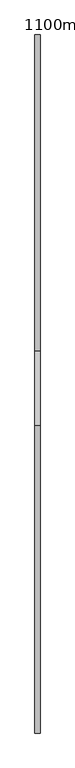
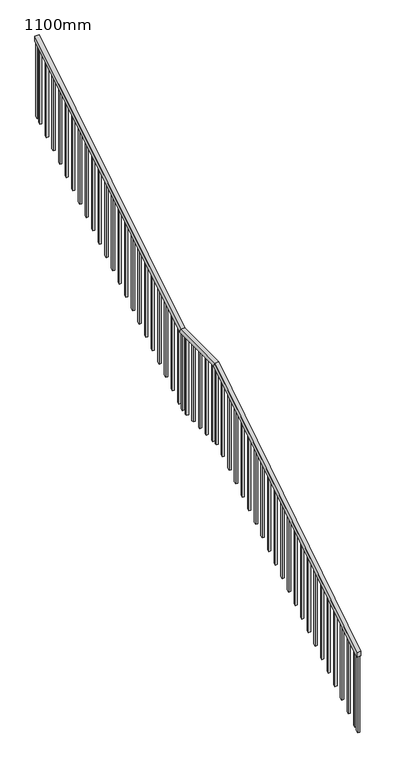
"""IFC4 building model written with IfcOpenShell, lengths in millimetres: railing geometry, 1100mm."""

import ifcopenshell
import ifcopenshell.guid

model = None  # the IFC model being written
_history = None  # IfcOwnerHistory: only IFC2X3 demands one
_inside = {}  # id of a spatial element -> (the spatial element, [elements in it])
_under = {}  # id of a project, library or spatial element -> (it, [spatial elements below it])
_declared = {}  # id of a project -> (the project, [libraries it declares])
_typed = {}  # id of a type object -> (the type object, [elements of that type])
_made_of = {}  # id of a material, layer set ... -> (it, [elements and type objects made of it])


def new_model(schema):
    """Start an empty IFC model of exactly this schema.

    Asked for "IFC4X3", IfcOpenShell would pick the latest addendum, in which some entities
    have other attributes; the version numbers below select the first issue.
    IFC2X3 requires an IfcOwnerHistory on every rooted entity: one is made here for all.
    """
    global model, _history
    if schema == "IFC4X3":
        model = ifcopenshell.file(schema_version=(4, 3, 0, 0))
    else:
        model = ifcopenshell.file(schema=schema)
    _inside.clear()
    _under.clear()
    _declared.clear()
    _typed.clear()
    _made_of.clear()
    _history = None
    if model.schema == "IFC2X3":
        org = make("IfcOrganization", Name="unknown")
        user = make(
            "IfcPersonAndOrganization",
            ThePerson=make("IfcPerson", FamilyName="unknown"),
            TheOrganization=org,
        )
        app = make(
            "IfcApplication",
            ApplicationDeveloper=org,
            Version="unknown",
            ApplicationFullName="unknown",
            ApplicationIdentifier="unknown",
        )
        _history = make(
            "IfcOwnerHistory",
            OwningUser=user,
            OwningApplication=app,
            ChangeAction="ADDED",
            CreationDate=0,
        )
    return model


def make(cls, **values):
    """One entity of the class cls with the attributes given. An attribute that is None is left unset."""
    return model.create_entity(
        cls, **{name: value for name, value in values.items() if value is not None}
    )


def rooted(cls, **values):
    """An entity with a GlobalId (a new one), such as an element, a storey or a relation."""
    return make(cls, GlobalId=ifcopenshell.guid.new(), OwnerHistory=_history, **values)


def si_unit(unit_type, name, prefix=None):
    """IfcSIUnit, for example si_unit("LENGTHUNIT", "METRE", prefix="MILLI")."""
    return make("IfcSIUnit", UnitType=unit_type, Prefix=prefix, Name=name)


def assignment(units):
    """IfcUnitAssignment: the units of a project."""
    return None if units is None else make("IfcUnitAssignment", Units=units)


def point(xyz):
    """IfcCartesianPoint."""
    return None if xyz is None else make("IfcCartesianPoint", Coordinates=xyz)


def direction(xyz):
    """IfcDirection."""
    return None if xyz is None else make("IfcDirection", DirectionRatios=xyz)


def frame(location, z_axis=None, x_axis=None):
    """IfcAxis2Placement3D, a coordinate frame: its origin and axes. An axis left out is left unset."""
    return make(
        "IfcAxis2Placement3D",
        Location=point(location),
        Axis=direction(z_axis),
        RefDirection=direction(x_axis),
    )


def origin():
    """The frame at (0, 0, 0) with its axes left unset."""
    return frame((0.0, 0.0, 0.0))


def place(relative_to, where):
    """IfcLocalPlacement: puts the frame where relative to a parent placement (None: the world)."""
    return make(
        "IfcLocalPlacement", PlacementRelTo=relative_to, RelativePlacement=where
    )


def context(
    kind, dimensions, precision=None, world=None, true_north=None, identifier=None
):
    """IfcGeometricRepresentationContext, for example the 3D "Model" context."""
    return make(
        "IfcGeometricRepresentationContext",
        ContextIdentifier=identifier,
        ContextType=kind,
        CoordinateSpaceDimension=dimensions,
        Precision=precision,
        WorldCoordinateSystem=world,
        TrueNorth=true_north,
    )


def project(units=None, contexts=None):
    """IfcProject with its units and contexts."""
    return rooted(
        "IfcProject",
        Name="project",
        RepresentationContexts=contexts,
        UnitsInContext=assignment(units),
    )


def spatial(cls, under=None, at=None, **own):
    """A site, building, storey or space (cls), placed at a placement, below another one or the project."""
    s = rooted(cls, ObjectPlacement=at, **own)
    if under is not None:
        _under.setdefault(under.id(), (under, []))[1].append(s)
    return s


def polyline(points):
    """IfcPolyline through the points."""
    return make("IfcPolyline", Points=[point(p) for p in points])


def outline(outer, holes=None, kind="AREA"):
    """IfcArbitraryClosedProfileDef: a profile drawn as a closed curve; with holes, ...WithVoids."""
    if holes is None:
        return make("IfcArbitraryClosedProfileDef", ProfileType=kind, OuterCurve=outer)
    return make(
        "IfcArbitraryProfileDefWithVoids",
        ProfileType=kind,
        OuterCurve=outer,
        InnerCurves=holes,
    )


def extrude(swept, where, along, depth):
    """IfcExtrudedAreaSolid: the profile swept, set in the frame where, extruded along a direction by depth."""
    return make(
        "IfcExtrudedAreaSolid",
        SweptArea=swept,
        Position=where,
        ExtrudedDirection=direction(along),
        Depth=depth,
    )


def faces_of(points, faces, orient=None, outer=None):
    """IfcFace entities. A face is a list of loops; a loop is a list of indices into points, from 0.

    orient and outer hold one flag for each loop. By default every Orientation is true, the
    first loop of a face is its IfcFaceOuterBound and the others are IfcFaceBound.
    """
    made = []
    for i, loops in enumerate(faces):
        bounds = []
        for j, loop in enumerate(loops):
            is_outer = j == 0 if outer is None else outer[i][j]
            bounds.append(
                make(
                    "IfcFaceOuterBound" if is_outer else "IfcFaceBound",
                    Bound=make("IfcPolyLoop", Polygon=[points[k] for k in loop]),
                    Orientation=True if orient is None else orient[i][j],
                )
            )
        made.append(make("IfcFace", Bounds=bounds))
    return made


def faceted_brep(points, faces, orient=None, outer=None, voids=None):
    """IfcFacetedBrep: a solid bounded by flat faces; with voids (closed shells), ...WithVoids."""
    shared = [point(p) for p in points]
    hull = make("IfcClosedShell", CfsFaces=faces_of(shared, faces, orient, outer))
    if voids is None:
        return make("IfcFacetedBrep", Outer=hull)
    return make(
        "IfcFacetedBrepWithVoids",
        Outer=hull,
        Voids=[
            make(cls, CfsFaces=faces_of(shared, fs, o, b)) for cls, fs, o, b in voids
        ],
    )


def shape(context_of_items, identifier, shape_type, items):
    """IfcShapeRepresentation: the items that make up one representation, for example the "Body"."""
    return make(
        "IfcShapeRepresentation",
        ContextOfItems=context_of_items,
        RepresentationIdentifier=identifier,
        RepresentationType=shape_type,
        Items=items,
    )


def source(mapping_origin, context_of_items, identifier, shape_type, items):
    """IfcRepresentationMap: a shape defined once, which mapped items show again and again."""
    return make(
        "IfcRepresentationMap",
        MappingOrigin=mapping_origin,
        MappedRepresentation=shape(context_of_items, identifier, shape_type, items),
    )


def transform(
    local_origin,
    x_axis=None,
    y_axis=None,
    z_axis=None,
    scale=None,
    scale2=None,
    scale3=None,
    uniform=True,
):
    """IfcCartesianTransformationOperator3D, or its non-uniform kind. x_axis, y_axis, z_axis: its Axis1, 2, 3."""
    if uniform:
        return make(
            "IfcCartesianTransformationOperator3D",
            Axis1=direction(x_axis),
            Axis2=direction(y_axis),
            LocalOrigin=point(local_origin),
            Scale=scale,
            Axis3=direction(z_axis),
        )
    return make(
        "IfcCartesianTransformationOperator3DnonUniform",
        Axis1=direction(x_axis),
        Axis2=direction(y_axis),
        LocalOrigin=point(local_origin),
        Scale=scale,
        Axis3=direction(z_axis),
        Scale2=scale2,
        Scale3=scale3,
    )


def mapped(mapping_source, mapping_target):
    """IfcMappedItem: shows the shape of a source again, moved by a transform."""
    return make(
        "IfcMappedItem", MappingSource=mapping_source, MappingTarget=mapping_target
    )


def made_of(thing, what):
    """Note that an element or type object is made of a material, layer set ...; save() writes the relation."""
    if what is not None:
        _made_of.setdefault(what.id(), (what, []))[1].append(thing)
    return thing


def element(
    cls,
    number,
    at=None,
    inside=None,
    cuts=None,
    type_object=None,
    material=None,
    context=None,
    identifier="Body",
    shape_type=None,
    held_by="IfcProductDefinitionShape",
    body=None,
    shapes=None,
    **own,
):
    """One element of the class cls, such as IfcWall. Its Tag is "e" and its number.

    at: its placement. inside: the storey or other place that contains it. cuts: it is an
    opening in that element (IfcRelVoidsElement). A single representation is given by context,
    identifier, shape_type and body (its items); several are given by shapes. held_by: the class
    of the entity that holds the representations. save() writes the other relations.
    """
    e = rooted(cls, Tag="e%d" % number, ObjectPlacement=at, **own)
    if body is not None:
        shapes = [shape(context, identifier, shape_type, body)]
    if shapes is not None:
        e.Representation = make(held_by, Representations=shapes)
    if inside is not None:
        _inside.setdefault(inside.id(), (inside, []))[1].append(e)
    if cuts is not None:
        rooted(
            "IfcRelVoidsElement", RelatingBuildingElement=cuts, RelatedOpeningElement=e
        )
    if type_object is not None:
        _typed.setdefault(type_object.id(), (type_object, []))[1].append(e)
    return made_of(e, material)


def aggregate(whole, parts):
    """IfcRelAggregates: a whole, such as a stair, and the parts it consists of."""
    return rooted("IfcRelAggregates", RelatingObject=whole, RelatedObjects=parts)


def save(model, path):
    """Write the relations noted so far, then the file.

    IfcRelAggregates (storeys below a building ...), IfcRelContainedInSpatialStructure (elements
    in a storey), IfcRelDefinesByType, IfcRelAssociatesMaterial and IfcRelDeclares: one each for
    every whole, place, type object, material and project.
    """
    for whole, parts in _under.values():
        aggregate(whole, parts)
    for where, things in _inside.values():
        rooted(
            "IfcRelContainedInSpatialStructure",
            RelatedElements=things,
            RelatingStructure=where,
        )
    for kind, things in _typed.values():
        rooted("IfcRelDefinesByType", RelatedObjects=things, RelatingType=kind)
    for what, things in _made_of.values():
        rooted("IfcRelAssociatesMaterial", RelatedObjects=things, RelatingMaterial=what)
    for by, libraries in _declared.values():
        rooted("IfcRelDeclares", RelatingContext=by, RelatedDefinitions=libraries)
    model.write(path)


def railing_1100mm_2fb11b6b(model_context):
    return source(origin(), model_context, "Body", "SolidModel", [
        faceted_brep([(-22150.0159097, -6684.456375, 1268.797954), (-22150.0159097, -6684.456375, 1209.4512039), (-22100.0159097, -6684.456375, 1209.4512039), (-22100.0159097, -6684.456375, 1268.797954), (-22150.0159097, -3684.456375, 3186.9565217), (-22150.0159097, -3669.8380579, 3136.9565217), (-22100.0159097, -3669.8380579, 3136.9565217), (-22100.0159097, -3684.456375, 3186.9565217), (-22150.0159097, -2964.456375, 3186.9565217), (-22150.0159097, -2950.192194, 3136.9565217), (-22100.0159097, -2950.192194, 3136.9565217), (-22100.0159097, -2964.456375, 3186.9565217), (-22150.0159097, 115.543625, 5100.0), (-22100.0159097, 115.543625, 5100.0), (-22100.0159097, 115.543625, 5041.1402603), (-22150.0159097, 115.543625, 5041.1402603)], [[[0, 1, 2, 3]], [[1, 0, 4, 5]], [[2, 1, 5, 6]], [[3, 2, 6, 7]], [[0, 3, 7, 4]], [[5, 4, 8, 9]], [[6, 5, 9, 10]], [[7, 6, 10, 11]], [[4, 7, 11, 8]], [[12, 13, 14, 15]], [[9, 8, 12, 15]], [[10, 9, 15, 14]], [[11, 10, 14, 13]], [[8, 11, 13, 12]]]),
        extrude(outline(polyline([(33.043625, 4989.8980242), (58.043625, 5005.4259745), (58.043625, 4024.5530048), (33.043625, 4009.0250545), (33.043625, 4989.8980242)])), frame((-22137.5159097, 0.0, 0.0), z_axis=(1.0, 0.0, 0.0), x_axis=(0.0, 1.0, 0.0)), (0.0, 0.0, 1.0), 25.0),
        extrude(outline(polyline([(-106.956375, 4902.9415025), (-81.956375, 4918.4694528), (-81.956375, 3937.5964831), (-106.956375, 3922.0685328), (-106.956375, 4902.9415025)])), frame((-22137.5159097, 0.0, 0.0), z_axis=(1.0, 0.0, 0.0), x_axis=(0.0, 1.0, 0.0)), (0.0, 0.0, 1.0), 25.0),
        extrude(outline(polyline([(-246.956375, 4815.9849807), (-221.956375, 4831.5129311), (-221.956375, 3850.6399613), (-246.956375, 3835.112011), (-246.956375, 4815.9849807)])), frame((-22137.5159097, 0.0, 0.0), z_axis=(1.0, 0.0, 0.0), x_axis=(0.0, 1.0, 0.0)), (0.0, 0.0, 1.0), 25.0),
        extrude(outline(polyline([(-386.956375, 4729.028459), (-361.956375, 4744.5564093), (-361.956375, 3763.6834396), (-386.956375, 3748.1554893), (-386.956375, 4729.028459)])), frame((-22137.5159097, 0.0, 0.0), z_axis=(1.0, 0.0, 0.0), x_axis=(0.0, 1.0, 0.0)), (0.0, 0.0, 1.0), 25.0),
        extrude(outline(polyline([(-526.956375, 4642.0719373), (-501.956375, 4657.5998876), (-501.956375, 3676.7269179), (-526.956375, 3661.1989675), (-526.956375, 4642.0719373)])), frame((-22137.5159097, 0.0, 0.0), z_axis=(1.0, 0.0, 0.0), x_axis=(0.0, 1.0, 0.0)), (0.0, 0.0, 1.0), 25.0),
        extrude(outline(polyline([(-666.956375, 4555.1154155), (-641.956375, 4570.6433658), (-641.956375, 3589.7703961), (-666.956375, 3574.2424458), (-666.956375, 4555.1154155)])), frame((-22137.5159097, 0.0, 0.0), z_axis=(1.0, 0.0, 0.0), x_axis=(0.0, 1.0, 0.0)), (0.0, 0.0, 1.0), 25.0),
        extrude(outline(polyline([(-806.956375, 4468.1588938), (-781.956375, 4483.6868441), (-781.956375, 3502.8138744), (-806.956375, 3487.2859241), (-806.956375, 4468.1588938)])), frame((-22137.5159097, 0.0, 0.0), z_axis=(1.0, 0.0, 0.0), x_axis=(0.0, 1.0, 0.0)), (0.0, 0.0, 1.0), 25.0),
        extrude(outline(polyline([(-946.956375, 4381.2023721), (-921.956375, 4396.7303224), (-921.956375, 3415.8573526), (-946.956375, 3400.3294023), (-946.956375, 4381.2023721)])), frame((-22137.5159097, 0.0, 0.0), z_axis=(1.0, 0.0, 0.0), x_axis=(0.0, 1.0, 0.0)), (0.0, 0.0, 1.0), 25.0),
        extrude(outline(polyline([(-1086.956375, 4294.2458503), (-1061.956375, 4309.7738006), (-1061.956375, 3328.9008309), (-1086.956375, 3313.3728806), (-1086.956375, 4294.2458503)])), frame((-22137.5159097, 0.0, 0.0), z_axis=(1.0, 0.0, 0.0), x_axis=(0.0, 1.0, 0.0)), (0.0, 0.0, 1.0), 25.0),
        extrude(outline(polyline([(-1226.956375, 4207.2893286), (-1201.956375, 4222.8172789), (-1201.956375, 3241.9443092), (-1226.956375, 3226.4163588), (-1226.956375, 4207.2893286)])), frame((-22137.5159097, 0.0, 0.0), z_axis=(1.0, 0.0, 0.0), x_axis=(0.0, 1.0, 0.0)), (0.0, 0.0, 1.0), 25.0),
        extrude(outline(polyline([(-1366.956375, 4120.3328068), (-1341.956375, 4135.8607571), (-1341.956375, 3154.9877874), (-1366.956375, 3139.4598371), (-1366.956375, 4120.3328068)])), frame((-22137.5159097, 0.0, 0.0), z_axis=(1.0, 0.0, 0.0), x_axis=(0.0, 1.0, 0.0)), (0.0, 0.0, 1.0), 25.0),
        extrude(outline(polyline([(-1506.956375, 4033.3762851), (-1481.956375, 4048.9042354), (-1481.956375, 3068.0312657), (-1506.956375, 3052.5033154), (-1506.956375, 4033.3762851)])), frame((-22137.5159097, 0.0, 0.0), z_axis=(1.0, 0.0, 0.0), x_axis=(0.0, 1.0, 0.0)), (0.0, 0.0, 1.0), 25.0),
        extrude(outline(polyline([(-1646.956375, 3946.4197634), (-1621.956375, 3961.9477137), (-1621.956375, 2981.0747439), (-1646.956375, 2965.5467936), (-1646.956375, 3946.4197634)])), frame((-22137.5159097, 0.0, 0.0), z_axis=(1.0, 0.0, 0.0), x_axis=(0.0, 1.0, 0.0)), (0.0, 0.0, 1.0), 25.0),
        extrude(outline(polyline([(-1786.956375, 3859.4632416), (-1761.956375, 3874.9911919), (-1761.956375, 2894.1182222), (-1786.956375, 2878.5902719), (-1786.956375, 3859.4632416)])), frame((-22137.5159097, 0.0, 0.0), z_axis=(1.0, 0.0, 0.0), x_axis=(0.0, 1.0, 0.0)), (0.0, 0.0, 1.0), 25.0),
        extrude(outline(polyline([(-1926.956375, 3772.5067199), (-1901.956375, 3788.0346702), (-1901.956375, 2807.1617005), (-1926.956375, 2791.6337502), (-1926.956375, 3772.5067199)])), frame((-22137.5159097, 0.0, 0.0), z_axis=(1.0, 0.0, 0.0), x_axis=(0.0, 1.0, 0.0)), (0.0, 0.0, 1.0), 25.0),
        extrude(outline(polyline([(-2066.956375, 3685.5501981), (-2041.956375, 3701.0781484), (-2041.956375, 2720.2051787), (-2066.956375, 2704.6772284), (-2066.956375, 3685.5501981)])), frame((-22137.5159097, 0.0, 0.0), z_axis=(1.0, 0.0, 0.0), x_axis=(0.0, 1.0, 0.0)), (0.0, 0.0, 1.0), 25.0),
        extrude(outline(polyline([(-2206.956375, 3598.5936764), (-2181.956375, 3614.1216267), (-2181.956375, 2633.248657), (-2206.956375, 2617.7207067), (-2206.956375, 3598.5936764)])), frame((-22137.5159097, 0.0, 0.0), z_axis=(1.0, 0.0, 0.0), x_axis=(0.0, 1.0, 0.0)), (0.0, 0.0, 1.0), 25.0),
        extrude(outline(polyline([(-2346.956375, 3511.6371547), (-2321.956375, 3527.165105), (-2321.956375, 2546.2921352), (-2346.956375, 2530.7641849), (-2346.956375, 3511.6371547)])), frame((-22137.5159097, 0.0, 0.0), z_axis=(1.0, 0.0, 0.0), x_axis=(0.0, 1.0, 0.0)), (0.0, 0.0, 1.0), 25.0),
        extrude(outline(polyline([(-2486.956375, 3424.6806329), (-2461.956375, 3440.2085832), (-2461.956375, 2459.3356135), (-2486.956375, 2443.8076632), (-2486.956375, 3424.6806329)])), frame((-22137.5159097, 0.0, 0.0), z_axis=(1.0, 0.0, 0.0), x_axis=(0.0, 1.0, 0.0)), (0.0, 0.0, 1.0), 25.0),
        extrude(outline(polyline([(-2626.956375, 3337.7241112), (-2601.956375, 3353.2520615), (-2601.956375, 2372.3790918), (-2626.956375, 2356.8511415), (-2626.956375, 3337.7241112)])), frame((-22137.5159097, 0.0, 0.0), z_axis=(1.0, 0.0, 0.0), x_axis=(0.0, 1.0, 0.0)), (0.0, 0.0, 1.0), 25.0),
        extrude(outline(polyline([(-2766.956375, 3250.7675894), (-2741.956375, 3266.2955398), (-2741.956375, 2285.42257), (-2766.956375, 2269.8946197), (-2766.956375, 3250.7675894)])), frame((-22137.5159097, 0.0, 0.0), z_axis=(1.0, 0.0, 0.0), x_axis=(0.0, 1.0, 0.0)), (0.0, 0.0, 1.0), 25.0),
        extrude(outline(polyline([(-2906.956375, 3163.8110677), (-2881.956375, 3179.339018), (-2881.956375, 2198.4660483), (-2906.956375, 2182.938098), (-2906.956375, 3163.8110677)])), frame((-22137.5159097, 0.0, 0.0), z_axis=(1.0, 0.0, 0.0), x_axis=(0.0, 1.0, 0.0)), (0.0, 0.0, 1.0), 25.0),
        extrude(outline(polyline([(-22137.5159097, -3066.956375), (-22137.5159097, -3041.956375), (-22112.5159097, -3041.956375), (-22112.5159097, -3066.956375), (-22137.5159097, -3066.956375)])), frame((0.0, 0.0, 2133.5443962), z_axis=(0.0, 0.0, 1.0), x_axis=(1.0, 0.0, 0.0)), (0.0, 0.0, 1.0), 1003.4121256),
        extrude(outline(polyline([(-22137.5159097, -3206.956375), (-22137.5159097, -3181.956375), (-22112.5159097, -3181.956375), (-22112.5159097, -3206.956375), (-22137.5159097, -3206.956375)])), frame((0.0, 0.0, 2133.5443962), z_axis=(0.0, 0.0, 1.0), x_axis=(1.0, 0.0, 0.0)), (0.0, 0.0, 1.0), 1003.4121256),
        extrude(outline(polyline([(-22137.5159097, -3346.956375), (-22137.5159097, -3321.956375), (-22112.5159097, -3321.956375), (-22112.5159097, -3346.956375), (-22137.5159097, -3346.956375)])), frame((0.0, 0.0, 2133.5443962), z_axis=(0.0, 0.0, 1.0), x_axis=(1.0, 0.0, 0.0)), (0.0, 0.0, 1.0), 1003.4121256),
        extrude(outline(polyline([(-22137.5159097, -3486.956375), (-22137.5159097, -3461.956375), (-22112.5159097, -3461.956375), (-22112.5159097, -3486.956375), (-22137.5159097, -3486.956375)])), frame((0.0, 0.0, 2133.5443962), z_axis=(0.0, 0.0, 1.0), x_axis=(1.0, 0.0, 0.0)), (0.0, 0.0, 1.0), 1003.4121256),
        extrude(outline(polyline([(-22137.5159097, -3626.956375), (-22137.5159097, -3601.956375), (-22112.5159097, -3601.956375), (-22112.5159097, -3626.956375), (-22137.5159097, -3626.956375)])), frame((0.0, 0.0, 2133.5443962), z_axis=(0.0, 0.0, 1.0), x_axis=(1.0, 0.0, 0.0)), (0.0, 0.0, 1.0), 1003.4121256),
        extrude(outline(polyline([(-3826.956375, 3036.4972397), (-3801.956375, 3052.4818944), (-3801.956375, 2074.2831542), (-3826.956375, 2058.2984994), (-3826.956375, 3036.4972397)])), frame((-22137.5159097, 0.0, 0.0), z_axis=(1.0, 0.0, 0.0), x_axis=(0.0, 1.0, 0.0)), (0.0, 0.0, 1.0), 25.0),
        extrude(outline(polyline([(-3966.956375, 2946.9831732), (-3941.956375, 2962.9678279), (-3941.956375, 1984.7690877), (-3966.956375, 1968.7844329), (-3966.956375, 2946.9831732)])), frame((-22137.5159097, 0.0, 0.0), z_axis=(1.0, 0.0, 0.0), x_axis=(0.0, 1.0, 0.0)), (0.0, 0.0, 1.0), 25.0),
        extrude(outline(polyline([(-4106.956375, 2857.4691067), (-4081.956375, 2873.4537614), (-4081.956375, 1895.2550212), (-4106.956375, 1879.2703664), (-4106.956375, 2857.4691067)])), frame((-22137.5159097, 0.0, 0.0), z_axis=(1.0, 0.0, 0.0), x_axis=(0.0, 1.0, 0.0)), (0.0, 0.0, 1.0), 25.0),
        extrude(outline(polyline([(-4246.956375, 2767.9550402), (-4221.956375, 2783.9396949), (-4221.956375, 1805.7409547), (-4246.956375, 1789.7562999), (-4246.956375, 2767.9550402)])), frame((-22137.5159097, 0.0, 0.0), z_axis=(1.0, 0.0, 0.0), x_axis=(0.0, 1.0, 0.0)), (0.0, 0.0, 1.0), 25.0),
        extrude(outline(polyline([(-4386.956375, 2678.4409737), (-4361.956375, 2694.4256284), (-4361.956375, 1716.2268882), (-4386.956375, 1700.2422334), (-4386.956375, 2678.4409737)])), frame((-22137.5159097, 0.0, 0.0), z_axis=(1.0, 0.0, 0.0), x_axis=(0.0, 1.0, 0.0)), (0.0, 0.0, 1.0), 25.0),
        extrude(outline(polyline([(-4526.956375, 2588.9269072), (-4501.956375, 2604.9115619), (-4501.956375, 1626.7128217), (-4526.956375, 1610.7281669), (-4526.956375, 2588.9269072)])), frame((-22137.5159097, 0.0, 0.0), z_axis=(1.0, 0.0, 0.0), x_axis=(0.0, 1.0, 0.0)), (0.0, 0.0, 1.0), 25.0),
        extrude(outline(polyline([(-4666.956375, 2499.4128407), (-4641.956375, 2515.3974954), (-4641.956375, 1537.1987552), (-4666.956375, 1521.2141004), (-4666.956375, 2499.4128407)])), frame((-22137.5159097, 0.0, 0.0), z_axis=(1.0, 0.0, 0.0), x_axis=(0.0, 1.0, 0.0)), (0.0, 0.0, 1.0), 25.0),
        extrude(outline(polyline([(-4806.956375, 2409.8987742), (-4781.956375, 2425.8834289), (-4781.956375, 1447.6846887), (-4806.956375, 1431.700034), (-4806.956375, 2409.8987742)])), frame((-22137.5159097, 0.0, 0.0), z_axis=(1.0, 0.0, 0.0), x_axis=(0.0, 1.0, 0.0)), (0.0, 0.0, 1.0), 25.0),
        extrude(outline(polyline([(-4946.956375, 2320.3847077), (-4921.956375, 2336.3693624), (-4921.956375, 1358.1706222), (-4946.956375, 1342.1859675), (-4946.956375, 2320.3847077)])), frame((-22137.5159097, 0.0, 0.0), z_axis=(1.0, 0.0, 0.0), x_axis=(0.0, 1.0, 0.0)), (0.0, 0.0, 1.0), 25.0),
        extrude(outline(polyline([(-5086.956375, 2230.8706412), (-5061.956375, 2246.8552959), (-5061.956375, 1268.6565557), (-5086.956375, 1252.671901), (-5086.956375, 2230.8706412)])), frame((-22137.5159097, 0.0, 0.0), z_axis=(1.0, 0.0, 0.0), x_axis=(0.0, 1.0, 0.0)), (0.0, 0.0, 1.0), 25.0),
        extrude(outline(polyline([(-5226.956375, 2141.3565747), (-5201.956375, 2157.3412294), (-5201.956375, 1179.1424892), (-5226.956375, 1163.1578345), (-5226.956375, 2141.3565747)])), frame((-22137.5159097, 0.0, 0.0), z_axis=(1.0, 0.0, 0.0), x_axis=(0.0, 1.0, 0.0)), (0.0, 0.0, 1.0), 25.0),
        extrude(outline(polyline([(-5366.956375, 2051.8425082), (-5341.956375, 2067.8271629), (-5341.956375, 1089.6284227), (-5366.956375, 1073.643768), (-5366.956375, 2051.8425082)])), frame((-22137.5159097, 0.0, 0.0), z_axis=(1.0, 0.0, 0.0), x_axis=(0.0, 1.0, 0.0)), (0.0, 0.0, 1.0), 25.0),
        extrude(outline(polyline([(-5506.956375, 1962.3284417), (-5481.956375, 1978.3130964), (-5481.956375, 1000.1143562), (-5506.956375, 984.1297015), (-5506.956375, 1962.3284417)])), frame((-22137.5159097, 0.0, 0.0), z_axis=(1.0, 0.0, 0.0), x_axis=(0.0, 1.0, 0.0)), (0.0, 0.0, 1.0), 25.0),
        extrude(outline(polyline([(-5646.956375, 1872.8143752), (-5621.956375, 1888.79903), (-5621.956375, 910.6002897), (-5646.956375, 894.615635), (-5646.956375, 1872.8143752)])), frame((-22137.5159097, 0.0, 0.0), z_axis=(1.0, 0.0, 0.0), x_axis=(0.0, 1.0, 0.0)), (0.0, 0.0, 1.0), 25.0),
        extrude(outline(polyline([(-5786.956375, 1783.3003087), (-5761.956375, 1799.2849635), (-5761.956375, 821.0862232), (-5786.956375, 805.1015685), (-5786.956375, 1783.3003087)])), frame((-22137.5159097, 0.0, 0.0), z_axis=(1.0, 0.0, 0.0), x_axis=(0.0, 1.0, 0.0)), (0.0, 0.0, 1.0), 25.0),
        extrude(outline(polyline([(-5926.956375, 1693.7862422), (-5901.956375, 1709.770897), (-5901.956375, 731.5721567), (-5926.956375, 715.587502), (-5926.956375, 1693.7862422)])), frame((-22137.5159097, 0.0, 0.0), z_axis=(1.0, 0.0, 0.0), x_axis=(0.0, 1.0, 0.0)), (0.0, 0.0, 1.0), 25.0),
        extrude(outline(polyline([(-6066.956375, 1604.2721757), (-6041.956375, 1620.2568305), (-6041.956375, 642.0580902), (-6066.956375, 626.0734355), (-6066.956375, 1604.2721757)])), frame((-22137.5159097, 0.0, 0.0), z_axis=(1.0, 0.0, 0.0), x_axis=(0.0, 1.0, 0.0)), (0.0, 0.0, 1.0), 25.0),
        extrude(outline(polyline([(-6206.956375, 1514.7581092), (-6181.956375, 1530.742764), (-6181.956375, 552.5440237), (-6206.956375, 536.559369), (-6206.956375, 1514.7581092)])), frame((-22137.5159097, 0.0, 0.0), z_axis=(1.0, 0.0, 0.0), x_axis=(0.0, 1.0, 0.0)), (0.0, 0.0, 1.0), 25.0),
        extrude(outline(polyline([(-6346.956375, 1425.2440427), (-6321.956375, 1441.2286975), (-6321.956375, 463.0299572), (-6346.956375, 447.0453025), (-6346.956375, 1425.2440427)])), frame((-22137.5159097, 0.0, 0.0), z_axis=(1.0, 0.0, 0.0), x_axis=(0.0, 1.0, 0.0)), (0.0, 0.0, 1.0), 25.0),
        extrude(outline(polyline([(-6486.956375, 1335.7299762), (-6461.956375, 1351.714631), (-6461.956375, 373.5158907), (-6486.956375, 357.531236), (-6486.956375, 1335.7299762)])), frame((-22137.5159097, 0.0, 0.0), z_axis=(1.0, 0.0, 0.0), x_axis=(0.0, 1.0, 0.0)), (0.0, 0.0, 1.0), 25.0),
        extrude(outline(polyline([(-6626.956375, 1246.2159097), (-6601.956375, 1262.2005645), (-6601.956375, 284.0018242), (-6626.956375, 268.0171695), (-6626.956375, 1246.2159097)])), frame((-22137.5159097, 0.0, 0.0), z_axis=(1.0, 0.0, 0.0), x_axis=(0.0, 1.0, 0.0)), (0.0, 0.0, 1.0), 25.0),
        extrude(outline(polyline([(-2976.956375, 3136.9565217), (-2951.956375, 3136.9565217), (-2951.956375, 2154.9877874), (-2976.956375, 2139.4598371), (-2976.956375, 3136.9565217)])), frame((-22137.5159097, 0.0, 0.0), z_axis=(1.0, 0.0, 0.0), x_axis=(0.0, 1.0, 0.0)), (0.0, 0.0, 1.0), 25.0),
        extrude(outline(polyline([(-3696.956375, 3119.6174443), (-3671.956375, 3135.602099), (-3671.956375, 2133.5443962), (-3696.956375, 2133.5443962), (-3696.956375, 3119.6174443)])), frame((-22137.5159097, 0.0, 0.0), z_axis=(1.0, 0.0, 0.0), x_axis=(0.0, 1.0, 0.0)), (0.0, 0.0, 1.0), 25.0),
        extrude(outline(polyline([(90.543625, 5025.6123099), (115.543625, 5041.1402603), (115.543625, 4060.2672905), (90.543625, 4044.7393402), (90.543625, 5025.6123099)])), frame((-22137.5159097, 0.0, 0.0), z_axis=(1.0, 0.0, 0.0), x_axis=(0.0, 1.0, 0.0)), (0.0, 0.0, 1.0), 25.0),
        extrude(outline(polyline([(-6684.456375, 1209.4512039), (-6659.456375, 1225.4358586), (-6659.456375, 247.2371184), (-6684.456375, 231.2524636), (-6684.456375, 1209.4512039)])), frame((-22137.5159097, 0.0, 0.0), z_axis=(1.0, 0.0, 0.0), x_axis=(0.0, 1.0, 0.0)), (0.0, 0.0, 1.0), 25.0),
    ])


if __name__ == "__main__":
    model = new_model("IFC4")
    model_context = context("Model", 3, world=origin())
    ifc_project = project(units=[si_unit("LENGTHUNIT", "METRE", prefix="MILLI")], contexts=[model_context])
    site = spatial("IfcSite", under=ifc_project)
    building = spatial("IfcBuilding", under=site)
    placement = place(None, origin())
    railing_1100mm_shape = railing_1100mm_2fb11b6b(model_context)
    element("IfcRailing", 1, ObjectType="1100mm", at=placement, inside=building, context=model_context, shape_type="MappedRepresentation", body=[
        mapped(railing_1100mm_shape, transform((0.0, 0.0, 0.0), x_axis=(1.0, 0.0, 0.0), y_axis=(0.0, 1.0, 0.0), z_axis=(0.0, 0.0, 1.0))),
    ])
    save(model, "model.ifc")
